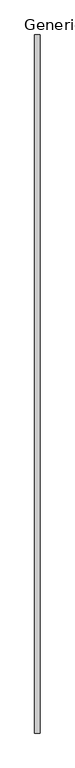
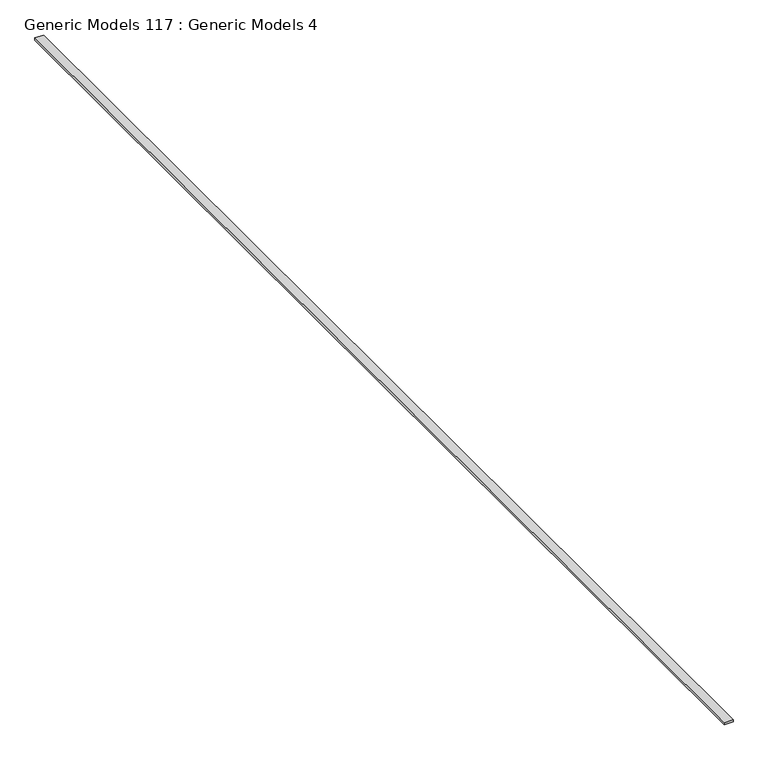
"""IFC4 building model written with IfcOpenShell, lengths in millimetres: proxy geometry, Generic Models 117 : Generic Models 4."""

from ifc_helpers import new_model, si_unit, frame, origin, place, context, project, spatial, polyline, outline, extrude, source, transform, mapped, element, save


def generic_models_117_generic_models_4_e9e49028(model_context):
    return source(origin(), model_context, "Body", "SweptSolid", [
        extrude(outline(polyline([(127066.3735933, 7095.9513704), (127066.3735933, 7235.6513704), (127098.6527599, 7235.6513704), (127104.4735933, 7095.9513704), (127066.3735933, 7095.9513704)])), frame((0.0, -6864.9230338, 0.0), z_axis=(0.0, 1.0, 0.0), x_axis=(0.0, 0.0, 1.0)), (0.0, 0.0, 1.0), 18643.6),
    ])


if __name__ == "__main__":
    model = new_model("IFC4")
    model_context = context("Model", 3, world=origin())
    ifc_project = project(units=[si_unit("LENGTHUNIT", "METRE", prefix="MILLI")], contexts=[model_context])
    site = spatial("IfcSite", under=ifc_project)
    building = spatial("IfcBuilding", under=site)
    placement = place(None, origin())
    generic_models_117_generic_models_4_shape = generic_models_117_generic_models_4_e9e49028(model_context)
    element("IfcBuildingElementProxy", 1, Name="Generic Models 117 : Generic Models 4", ObjectType="Generic Models 117 : Generic Models 4", at=placement, inside=building, context=model_context, shape_type="MappedRepresentation", body=[
        mapped(generic_models_117_generic_models_4_shape, transform((0.0, 0.0, 0.0), x_axis=(1.0, 0.0, 0.0), y_axis=(0.0, 1.0, 0.0), z_axis=(0.0, 0.0, 1.0))),
    ])
    save(model, "model.ifc")

# Revit data of these elements
# Element 1 (IfcBuildingElementProxy, "Generic Models 117 : Generic Models 4")
#   Materials on its faces: "_2X BLOCKING AS REQUIRED"
# Materials
#   "_2X BLOCKING AS REQUIRED": class "Generic", colour RGB 177 130 114, transparency 0, Cost = 0
